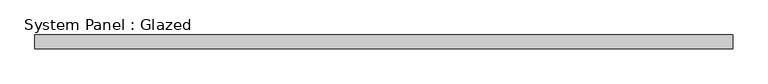
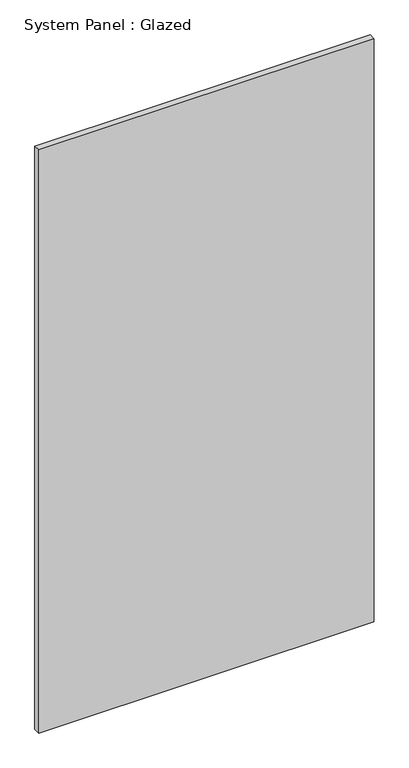
"""IFC4 building model written with IfcOpenShell, lengths in millimetres: plate geometry, System Panel : Glazed."""

from ifc_helpers import new_model, si_unit, origin, origin_with_axes, place, context, project, spatial, polyline, outline, extrude, source, transform, mapped, element, save


def system_panel_glazed_7be3c4b1(model_context):
    return source(origin(), model_context, "Body", "SweptSolid", [
        extrude(outline(polyline([(633.0541355, 24.5), (-633.0541355, 24.5), (-633.0541355, 49.5), (633.0541355, 49.5), (633.0541355, 24.5)])), origin_with_axes(), (0.0, 0.0, 1.0), 2325.0),
    ])


if __name__ == "__main__":
    model = new_model("IFC4")
    model_context = context("Model", 3, world=origin())
    ifc_project = project(units=[si_unit("LENGTHUNIT", "METRE", prefix="MILLI")], contexts=[model_context])
    site = spatial("IfcSite", under=ifc_project)
    building = spatial("IfcBuilding", under=site)
    placement = place(None, origin())
    system_panel_glazed_shape = system_panel_glazed_7be3c4b1(model_context)
    element("IfcPlate", 1, ObjectType="System Panel : Glazed", at=placement, inside=building, context=model_context, shape_type="MappedRepresentation", body=[
        mapped(system_panel_glazed_shape, transform((0.0, 0.0, 0.0), x_axis=(1.0, 0.0, 0.0), y_axis=(0.0, 1.0, 0.0), z_axis=(0.0, 0.0, 1.0))),
    ])
    save(model, "model.ifc")

# Revit data of these elements
# Type "System Panel : Glazed"
#   Construction Type Id = "GSP4R"
#   Analytic Construction = "1/8 in Pilkington single glazing"
#   Visual Light Transmittance = 0.9
#   Solar Heat Gain Coefficient = 0.86
#   Heat Transfer Coefficient (U) = 6.7069 W/(m²·K)
#   Define Thermal Properties by = 1
# Element 1 (IfcPlate, "System Panel : Glazed")
#   Materials on its faces: "Glass"
# Materials
#   "Glass": class "Glass", colour RGB 0 128 192, transparency 0.9, Description = "Soda Lime Glass", Cost = 0
